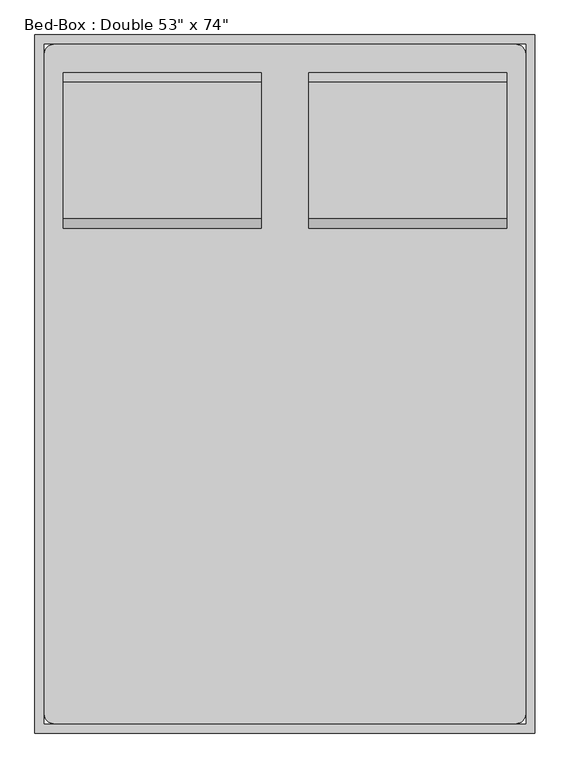
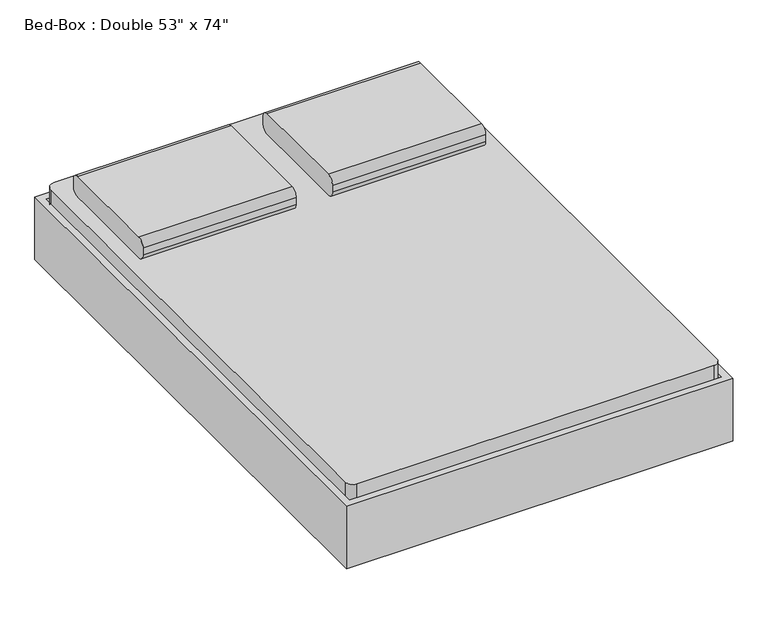
"""IFC4 building model written with IfcOpenShell, lengths in millimetres: furniture geometry."""

from ifc_helpers import new_model, si_unit, point, frame, frame_2d, origin, place, context, project, spatial, polyline, circle_curve, trimmed, segment, composite_curve, outline, extrude, source, transform, mapped, element, save
from ifc_brep_helpers import plane_surface, cylinder_surface, revolved_surface, advanced_brep


def furniture_bd6c971a(model_context):
    return source(origin(), model_context, "Body", "SolidModel", [
        extrude(outline(composite_curve([segment(polyline([(578.3704918, 406.4), (210.0704918, 406.4)]), True, "CONTINUOUS"), segment(trimmed(circle_curve(frame_2d((210.0704918, 431.8)), 25.4), [point((210.0704918, 406.4))], [point((184.6704918, 431.8))], False, "CARTESIAN"), True, "CONTINUOUS"), segment(polyline([(184.6704918, 431.8), (184.6704918, 457.2)]), True, "CONTINUOUS"), segment(trimmed(circle_curve(frame_2d((210.0704918, 457.2)), 25.4), [point((184.6704918, 457.2))], [point((210.0704918, 482.6))], False, "CARTESIAN"), True, "CONTINUOUS"), segment(polyline([(210.0704918, 482.6), (578.3704918, 482.6)]), True, "CONTINUOUS"), segment(trimmed(circle_curve(frame_2d((578.3704918, 457.2)), 25.4), [point((578.3704918, 482.6))], [point((603.7704918, 457.2))], False, "CARTESIAN"), True, "CONTINUOUS"), segment(polyline([(603.7704918, 457.2), (603.7704918, 431.8)]), True, "CONTINUOUS"), segment(trimmed(circle_curve(frame_2d((578.3704918, 431.8)), 25.4), [point((603.7704918, 431.8))], [point((578.3704918, 406.4))], False, "CARTESIAN"), True, "CONTINUOUS")], self_intersect=False)), frame((402.652459, 0.0, 0.0), z_axis=(1.0, 0.0, 0.0), x_axis=(0.0, 1.0, 0.0)), (0.0, 0.0, 1.0), 533.4),
        extrude(outline(composite_curve([segment(polyline([(578.3704918, 406.4), (210.0704918, 406.4)]), True, "CONTINUOUS"), segment(trimmed(circle_curve(frame_2d((210.0704918, 431.8)), 25.4), [point((210.0704918, 406.4))], [point((184.6704918, 431.8))], False, "CARTESIAN"), True, "CONTINUOUS"), segment(polyline([(184.6704918, 431.8), (184.6704918, 457.2)]), True, "CONTINUOUS"), segment(trimmed(circle_curve(frame_2d((210.0704918, 457.2)), 25.4), [point((184.6704918, 457.2))], [point((210.0704918, 482.6))], False, "CARTESIAN"), True, "CONTINUOUS"), segment(polyline([(210.0704918, 482.6), (578.3704918, 482.6)]), True, "CONTINUOUS"), segment(trimmed(circle_curve(frame_2d((578.3704918, 457.2)), 25.4), [point((578.3704918, 482.6))], [point((603.7704918, 457.2))], False, "CARTESIAN"), True, "CONTINUOUS"), segment(polyline([(603.7704918, 457.2), (603.7704918, 431.8)]), True, "CONTINUOUS"), segment(trimmed(circle_curve(frame_2d((578.3704918, 431.8)), 25.4), [point((603.7704918, 431.8))], [point((578.3704918, 406.4))], False, "CARTESIAN"), True, "CONTINUOUS")], self_intersect=False)), frame((-257.747541, 0.0, 0.0), z_axis=(1.0, 0.0, 0.0), x_axis=(0.0, 1.0, 0.0)), (0.0, 0.0, 1.0), 533.4),
        advanced_brep(
        [(-308.2231784, 451.3704918, 177.8), (-308.2231784, 375.1704918, 177.8), (-308.2231784, 375.1704918, 196.85), (-308.2231784, 451.3704918, 196.85), (-257.4231784, 451.3704918, 177.8), (-257.4231784, 375.1704918, 177.8), (-245.2869899, 375.1704918, 196.85), (-245.2869899, 451.3704918, 196.85), (-181.3523099, 451.3704918, 14.6654962), (-181.3523099, 375.1704918, 14.6654962), (-164.0871466, 375.1704918, 22.716374), (-164.0871466, 451.3704918, 22.716374), (-158.3320921, 375.1704918, 0.0), (-158.3320921, 451.3704918, 0.0), (-158.3320921, 375.1704918, 19.05), (-158.3320921, 451.3704918, 19.05), (-79.7195862, 451.3704918, 0.0), (-79.7195862, 375.1704918, 0.0), (-79.7195862, 375.1704918, 19.05), (-79.7195862, 451.3704918, 19.05), (-67.0195862, 375.1704918, 3.4029547), (-67.0195862, 451.3704918, 3.4029547), (-76.5445862, 375.1704918, 19.9007387), (-76.5445862, 451.3704918, 19.9007387), (-6.922541, 451.3704918, 38.1), (-6.922541, 375.1704918, 38.1), (-12.0269731, 375.1704918, 57.15), (-12.0269731, 451.3704918, 57.15), (685.5518216, 451.3704918, 38.1), (685.5518216, 375.1704918, 38.1), (690.6562537, 375.1704918, 57.15), (690.6562537, 451.3704918, 57.15), (745.6488669, 451.3704918, 3.4029547), (745.6488669, 375.1704918, 3.4029547), (755.1738669, 375.1704918, 19.9007387), (755.1738669, 451.3704918, 19.9007387), (758.3488669, 375.1704918, 0.0), (758.3488669, 451.3704918, 0.0), (758.3488669, 375.1704918, 19.05), (758.3488669, 451.3704918, 19.05), (836.9613728, 451.3704918, 0.0), (836.9613728, 375.1704918, 0.0), (836.9613728, 375.1704918, 19.05), (836.9613728, 451.3704918, 19.05), (859.9815906, 375.1704918, 14.6654962), (859.9815906, 451.3704918, 14.6654962), (842.7164272, 375.1704918, 22.716374), (842.7164272, 451.3704918, 22.716374), (936.052459, 451.3704918, 177.8), (936.052459, 375.1704918, 177.8), (923.9162705, 375.1704918, 196.85), (923.9162705, 451.3704918, 196.85), (986.852459, 451.3704918, 177.8), (986.852459, 451.3704918, 196.85), (986.852459, 375.1704918, 196.85), (986.852459, 375.1704918, 177.8)],
        [
            (0, 1),
            (1, 2),
            (2, 3),
            (3, 0),
            (0, 4),
            (4, 5),
            (5, 1),
            (5, 6),
            (6, 2),
            (6, 7),
            (7, 3),
            (7, 4),
            (4, 8),
            (8, 9),
            (9, 5),
            (9, 10),
            (10, 6),
            (10, 11),
            (11, 7),
            (11, 8),
            (12, 9, circle_curve(frame((-158.3320921, 375.1704918, 25.4), z_axis=(0.0, 1.0, 0.0), x_axis=(-0.9063077870366486, 0.0, -0.42261826174070233)), 25.4)),
            (8, 13, circle_curve(frame((-158.3320921, 451.3704918, 25.4), z_axis=(0.0, -1.0, 0.0), x_axis=(-0.9063077870366486, 0.0, -0.42261826174070233)), 25.4)),
            (13, 12),
            (14, 10, circle_curve(frame((-158.3320921, 375.1704918, 25.4), z_axis=(0.0, 1.0, 0.0), x_axis=(-0.9063077870366486, 0.0, -0.42261826174070233)), 6.35)),
            (12, 14),
            (15, 11, circle_curve(frame((-158.3320921, 451.3704918, 25.4), z_axis=(0.0, 1.0, 0.0), x_axis=(-0.9063077870366486, 0.0, -0.42261826174070233)), 6.35)),
            (14, 15),
            (15, 13),
            (13, 16),
            (16, 17),
            (17, 12),
            (17, 18),
            (18, 14),
            (18, 19),
            (19, 15),
            (19, 16),
            (20, 17, circle_curve(frame((-79.7195862, 375.1704918, 25.4), z_axis=(0.0, 1.0, 0.0), x_axis=(0.0, 0.0, -1.0)), 25.4)),
            (16, 21, circle_curve(frame((-79.7195862, 451.3704918, 25.4), z_axis=(0.0, -1.0, 0.0), x_axis=(0.0, 0.0, -1.0)), 25.4)),
            (21, 20),
            (22, 18, circle_curve(frame((-79.7195862, 375.1704918, 25.4), z_axis=(0.0, 1.0, 0.0), x_axis=(0.0, 0.0, -1.0)), 6.35)),
            (20, 22),
            (23, 19, circle_curve(frame((-79.7195862, 451.3704918, 25.4), z_axis=(0.0, 1.0, 0.0), x_axis=(0.0, 0.0, -1.0)), 6.35)),
            (22, 23),
            (23, 21),
            (21, 24),
            (24, 25),
            (25, 20),
            (25, 26),
            (26, 22),
            (26, 27),
            (27, 23),
            (27, 24),
            (24, 28),
            (28, 29),
            (29, 25),
            (29, 30),
            (30, 26),
            (30, 31),
            (31, 27),
            (31, 28),
            (28, 32),
            (32, 33),
            (33, 29),
            (33, 34),
            (34, 30),
            (34, 35),
            (35, 31),
            (35, 32),
            (36, 33, circle_curve(frame((758.3488669, 375.1704918, 25.4), z_axis=(0.0, 1.0, 0.0), x_axis=(-0.5000000000000463, 0.0, -0.8660254037844118)), 25.4)),
            (32, 37, circle_curve(frame((758.3488669, 451.3704918, 25.4), z_axis=(0.0, -1.0, 0.0), x_axis=(-0.5000000000000463, 0.0, -0.8660254037844118)), 25.4)),
            (37, 36),
            (38, 34, circle_curve(frame((758.3488669, 375.1704918, 25.4), z_axis=(0.0, 1.0, 0.0), x_axis=(-0.5000000000000463, 0.0, -0.8660254037844118)), 6.35)),
            (36, 38),
            (39, 35, circle_curve(frame((758.3488669, 451.3704918, 25.4), z_axis=(0.0, 1.0, 0.0), x_axis=(-0.5000000000000463, 0.0, -0.8660254037844118)), 6.35)),
            (38, 39),
            (39, 37),
            (37, 40),
            (40, 41),
            (41, 36),
            (41, 42),
            (42, 38),
            (42, 43),
            (43, 39),
            (43, 40),
            (44, 41, circle_curve(frame((836.9613728, 375.1704918, 25.4), z_axis=(0.0, 1.0, 0.0), x_axis=(0.0, 0.0, -1.0)), 25.4)),
            (40, 45, circle_curve(frame((836.9613728, 451.3704918, 25.4), z_axis=(0.0, -1.0, 0.0), x_axis=(0.0, 0.0, -1.0)), 25.4)),
            (45, 44),
            (46, 42, circle_curve(frame((836.9613728, 375.1704918, 25.4), z_axis=(0.0, 1.0, 0.0), x_axis=(0.0, 0.0, -1.0)), 6.35)),
            (44, 46),
            (47, 43, circle_curve(frame((836.9613728, 451.3704918, 25.4), z_axis=(0.0, 1.0, 0.0), x_axis=(0.0, 0.0, -1.0)), 6.35)),
            (46, 47),
            (47, 45),
            (45, 48),
            (48, 49),
            (49, 44),
            (49, 50),
            (50, 46),
            (50, 51),
            (51, 47),
            (51, 48),
            (52, 53),
            (53, 54),
            (54, 55),
            (55, 52),
            (48, 52),
            (55, 49),
            (54, 50),
            (53, 51),
        ],
        [
            plane_surface(frame((-308.2231784, 705.3704918, -152.9490627), z_axis=(-1.0, 0.0, 0.0), x_axis=(0.0, 1.0, 0.0))),
            plane_surface(frame((-308.2231784, 451.3704918, 177.8), z_axis=(0.0, 0.0, -1.0), x_axis=(1.0, 0.0, 0.0))),
            plane_surface(frame((-308.2231784, 375.1704918, 177.8), z_axis=(0.0, -1.0, 0.0), x_axis=(1.0, 0.0, 0.0))),
            plane_surface(frame((-308.2231784, 375.1704918, 196.85), z_axis=(0.0, 0.0, 1.0), x_axis=(1.0, 0.0, 0.0))),
            plane_surface(frame((-308.2231784, 451.3704918, 196.85), z_axis=(0.0, 1.0, 0.0), x_axis=(1.0, 0.0, 0.0))),
            plane_surface(frame((-257.4231784, 451.3704918, 177.8), z_axis=(-0.9063077870366488, 0.0, -0.42261826174070194), x_axis=(0.42261826174070194, 0.0, -0.9063077870366488))),
            plane_surface(frame((-257.4231784, 375.1704918, 177.8), z_axis=(0.0, -1.0, 0.0), x_axis=(0.42261826174070194, 0.0, -0.9063077870366488))),
            plane_surface(frame((-245.2869899, 375.1704918, 196.85), z_axis=(0.9063077870366487, 0.0, 0.4226182617407021), x_axis=(0.4226182617407021, 0.0, -0.9063077870366487))),
            plane_surface(frame((-245.2869899, 451.3704918, 196.85), z_axis=(0.0, 1.0, 0.0), x_axis=(0.4226182617407021, 0.0, -0.9063077870366487))),
            cylinder_surface(frame((-158.3320921, 705.3704918, 25.4), z_axis=(0.0, -1.0, 0.0), x_axis=(-0.9063077870366486, 0.0, -0.42261826174070233)), 25.4),
            plane_surface(frame((-158.3320921, 375.1704918, 25.4), z_axis=(0.0, -1.0, 0.0), x_axis=(-0.9063077870366486, 0.0, -0.42261826174070233))),
            revolved_surface(polyline([(-164.08714654768272, 375.1704918, 22.71637403794654), (-164.08714654768272, 451.3704918, 22.71637403794654)]), (-158.3320921, 705.3704918, 25.4), (0.0, -1.0, 0.0)),
            plane_surface(frame((-158.3320921, 451.3704918, 25.4), z_axis=(0.0, 1.0, 0.0), x_axis=(-0.9063077870366486, 0.0, -0.42261826174070233))),
            plane_surface(frame((-158.3320921, 451.3704918, 0.0), z_axis=(0.0, 0.0, -1.0), x_axis=(1.0, 0.0, 0.0))),
            plane_surface(frame((-158.3320921, 375.1704918, 0.0), z_axis=(0.0, -1.0, 0.0), x_axis=(1.0, 0.0, 0.0))),
            plane_surface(frame((-158.3320921, 375.1704918, 19.05), z_axis=(0.0, 0.0, 1.0), x_axis=(1.0, 0.0, 0.0))),
            plane_surface(frame((-158.3320921, 451.3704918, 19.05), z_axis=(0.0, 1.0, 0.0), x_axis=(1.0, 0.0, 0.0))),
            cylinder_surface(frame((-79.7195862, 705.3704918, 25.4), z_axis=(0.0, -1.0, 0.0), x_axis=(0.0, 0.0, -1.0)), 25.4),
            plane_surface(frame((-79.7195862, 375.1704918, 25.4), z_axis=(0.0, -1.0, 0.0), x_axis=(0.0, 0.0, -1.0))),
            revolved_surface(polyline([(-79.7195862, 375.1704918, 19.049999999999997), (-79.7195862, 451.3704918, 19.049999999999997)]), (-79.7195862, 705.3704918, 25.4), (0.0, -1.0, 0.0)),
            plane_surface(frame((-79.7195862, 451.3704918, 25.4), z_axis=(0.0, 1.0, 0.0), x_axis=(0.0, 0.0, -1.0))),
            plane_surface(frame((-67.0195862, 451.3704918, 3.4029547), z_axis=(0.4999999999998774, 0.0, -0.8660254037845095), x_axis=(0.8660254037845095, 0.0, 0.4999999999998774))),
            plane_surface(frame((-67.0195862, 375.1704918, 3.4029547), z_axis=(0.0, -1.0, 0.0), x_axis=(0.866025403784509, 0.0, 0.49999999999987815))),
            plane_surface(frame((-76.5445862, 375.1704918, 19.9007387), z_axis=(-0.49999999999987754, 0.0, 0.8660254037845093), x_axis=(0.8660254037845093, 0.0, 0.49999999999987754))),
            plane_surface(frame((-76.5445862, 451.3704918, 19.9007387), z_axis=(0.0, 1.0000000000000002, 0.0), x_axis=(0.8660254037845091, 0.0, 0.49999999999987815))),
            plane_surface(frame((-6.922541, 451.3704918, 38.1), z_axis=(0.0, 0.0, -1.0), x_axis=(1.0, 0.0, 0.0))),
            plane_surface(frame((-6.922541, 375.1704918, 38.1), z_axis=(0.0, -1.0, 0.0), x_axis=(1.0, 0.0, 0.0))),
            plane_surface(frame((-12.0269731, 375.1704918, 57.15), z_axis=(0.0, 0.0, 1.0), x_axis=(1.0, 0.0, 0.0))),
            plane_surface(frame((-12.0269731, 451.3704918, 57.15), z_axis=(0.0, 1.0, 0.0), x_axis=(1.0, 0.0, 0.0))),
            plane_surface(frame((685.5518216, 451.3704918, 38.1), z_axis=(-0.500000000000047, 0.0, -0.8660254037844115), x_axis=(0.8660254037844115, 0.0, -0.500000000000047))),
            plane_surface(frame((685.5518216, 375.1704918, 38.1), z_axis=(0.0, -1.0, 0.0), x_axis=(0.8660254037844116, 0.0, -0.500000000000047))),
            plane_surface(frame((690.6562537, 375.1704918, 57.15), z_axis=(0.5000000000000456, 0.0, 0.8660254037844124), x_axis=(0.8660254037844124, 0.0, -0.5000000000000456))),
            plane_surface(frame((690.6562537, 451.3704918, 57.15), z_axis=(0.0, 1.0, 0.0), x_axis=(0.8660254037844124, 0.0, -0.5000000000000456))),
            cylinder_surface(frame((758.3488669, 705.3704918, 25.4), z_axis=(0.0, -1.0, 0.0), x_axis=(-0.5000000000000463, 0.0, -0.8660254037844118)), 25.4),
            plane_surface(frame((758.3488669, 375.1704918, 25.4), z_axis=(0.0, -1.0000000000000002, 0.0), x_axis=(-0.5000000000000464, 0.0, -0.866025403784412))),
            revolved_surface(polyline([(755.1738668999997, 375.1704918, 19.90073868596898), (755.1738668999997, 451.3704918, 19.90073868596898)]), (758.3488669, 705.3704918, 25.4), (0.0, -1.0, 0.0)),
            plane_surface(frame((758.3488669, 451.3704918, 25.4), z_axis=(0.0, 1.0000000000000002, 0.0), x_axis=(-0.5000000000000464, 0.0, -0.866025403784412))),
            plane_surface(frame((758.3488669, 451.3704918, 0.0), z_axis=(0.0, 0.0, -1.0), x_axis=(1.0, 0.0, 0.0))),
            plane_surface(frame((758.3488669, 375.1704918, 0.0), z_axis=(0.0, -1.0, 0.0), x_axis=(1.0, 0.0, 0.0))),
            plane_surface(frame((758.3488669, 375.1704918, 19.05), z_axis=(0.0, 0.0, 1.0), x_axis=(1.0, 0.0, 0.0))),
            plane_surface(frame((758.3488669, 451.3704918, 19.05), z_axis=(0.0, 1.0, 0.0), x_axis=(1.0, 0.0, 0.0))),
            cylinder_surface(frame((836.9613728, 705.3704918, 25.4), z_axis=(0.0, -1.0, 0.0), x_axis=(0.0, 0.0, -1.0)), 25.4),
            plane_surface(frame((836.9613728, 375.1704918, 25.4), z_axis=(0.0, -1.0, 0.0), x_axis=(0.0, 0.0, -1.0))),
            revolved_surface(polyline([(836.9613728, 375.1704918, 19.049999999999997), (836.9613728, 451.3704918, 19.049999999999997)]), (836.9613728, 705.3704918, 25.4), (0.0, -1.0, 0.0)),
            plane_surface(frame((836.9613728, 451.3704918, 25.4), z_axis=(0.0, 1.0, 0.0), x_axis=(0.0, 0.0, -1.0))),
            plane_surface(frame((859.9815906, 451.3704918, 14.6654962), z_axis=(0.9063077870366798, 0.0, -0.4226182617406355), x_axis=(0.4226182617406355, 0.0, 0.9063077870366798))),
            plane_surface(frame((859.9815906, 375.1704918, 14.6654962), z_axis=(0.0, -1.0, 0.0), x_axis=(0.4226182617406356, 0.0, 0.9063077870366797))),
            plane_surface(frame((842.7164272, 375.1704918, 22.716374), z_axis=(-0.9063077870366797, 0.0, 0.4226182617406358), x_axis=(0.4226182617406358, 0.0, 0.9063077870366797))),
            plane_surface(frame((842.7164272, 451.3704918, 22.716374), z_axis=(0.0, 1.0000000000000002, 0.0), x_axis=(0.42261826174063544, 0.0, 0.9063077870366799))),
            plane_surface(frame((986.852459, 705.3704918, -152.9490627), z_axis=(1.0, 0.0, 0.0), x_axis=(0.0, 1.0, 0.0))),
            plane_surface(frame((936.052459, 451.3704918, 177.8), z_axis=(0.0, 0.0, -1.0), x_axis=(1.0, 0.0, 0.0))),
            plane_surface(frame((936.052459, 375.1704918, 177.8), z_axis=(0.0, -1.0, 0.0), x_axis=(1.0, 0.0, 0.0))),
            plane_surface(frame((923.9162705, 375.1704918, 196.85), z_axis=(0.0, 0.0, 1.0), x_axis=(1.0, 0.0, 0.0))),
            plane_surface(frame((923.9162705, 451.3704918, 196.85), z_axis=(0.0, 1.0, 0.0), x_axis=(1.0, 0.0, 0.0))),
        ],
        [
            (0, [[1, 2, 3, 4]]),
            (1, [[-1, 5, 6, 7]]),
            (2, [[-2, -7, 8, 9]]),
            (3, [[-3, -9, 10, 11]]),
            (4, [[-4, -11, 12, -5]]),
            (5, [[-6, 13, 14, 15]]),
            (6, [[-8, -15, 16, 17]]),
            (7, [[-10, -17, 18, 19]]),
            (8, [[-12, -19, 20, -13]]),
            (9, [[21, -14, 22, 23]]),
            (10, [[24, -16, -21, 25]]),
            (11, [[26, -18, -24, 27]]),
            (12, [[-22, -20, -26, 28]]),
            (13, [[-23, 29, 30, 31]]),
            (14, [[-25, -31, 32, 33]]),
            (15, [[-27, -33, 34, 35]]),
            (16, [[-28, -35, 36, -29]]),
            (17, [[37, -30, 38, 39]]),
            (18, [[40, -32, -37, 41]]),
            (19, [[42, -34, -40, 43]]),
            (20, [[-38, -36, -42, 44]]),
            (21, [[-39, 45, 46, 47]]),
            (22, [[-41, -47, 48, 49]]),
            (23, [[-43, -49, 50, 51]]),
            (24, [[-44, -51, 52, -45]]),
            (25, [[-46, 53, 54, 55]]),
            (26, [[-48, -55, 56, 57]]),
            (27, [[-50, -57, 58, 59]]),
            (28, [[-52, -59, 60, -53]]),
            (29, [[-54, 61, 62, 63]]),
            (30, [[-56, -63, 64, 65]]),
            (31, [[-58, -65, 66, 67]]),
            (32, [[-60, -67, 68, -61]]),
            (33, [[69, -62, 70, 71]]),
            (34, [[72, -64, -69, 73]]),
            (35, [[74, -66, -72, 75]]),
            (36, [[-70, -68, -74, 76]]),
            (37, [[-71, 77, 78, 79]]),
            (38, [[-73, -79, 80, 81]]),
            (39, [[-75, -81, 82, 83]]),
            (40, [[-76, -83, 84, -77]]),
            (41, [[85, -78, 86, 87]]),
            (42, [[88, -80, -85, 89]]),
            (43, [[90, -82, -88, 91]]),
            (44, [[-86, -84, -90, 92]]),
            (45, [[-87, 93, 94, 95]]),
            (46, [[-89, -95, 96, 97]]),
            (47, [[-91, -97, 98, 99]]),
            (48, [[-92, -99, 100, -93]]),
            (49, [[101, 102, 103, 104]]),
            (50, [[-94, 105, -104, 106]]),
            (51, [[-96, -106, -103, 107]]),
            (52, [[-98, -107, -102, 108]]),
            (53, [[-100, -108, -101, -105]]),
        ],
    ),
        extrude(outline(composite_curve([segment(polyline([(-283.147541, 679.9704918), (961.452459, 679.9704918)]), True, "CONTINUOUS"), segment(trimmed(circle_curve(frame_2d((961.452459, 654.5704918)), 25.4), [point((961.452459, 679.9704918))], [point((986.852459, 654.5704918))], False, "CARTESIAN"), True, "CONTINUOUS"), segment(polyline([(986.852459, 654.5704918), (986.852459, -1123.4295082)]), True, "CONTINUOUS"), segment(trimmed(circle_curve(frame_2d((961.452459, -1123.4295082)), 25.4), [point((986.852459, -1123.4295082))], [point((961.452459, -1148.8295082))], False, "CARTESIAN"), True, "CONTINUOUS"), segment(polyline([(961.452459, -1148.8295082), (-283.147541, -1148.8295082)]), True, "CONTINUOUS"), segment(trimmed(circle_curve(frame_2d((-283.147541, -1123.4295082)), 25.4), [point((-283.147541, -1148.8295082))], [point((-308.547541, -1123.4295082))], False, "CARTESIAN"), True, "CONTINUOUS"), segment(polyline([(-308.547541, -1123.4295082), (-308.547541, 654.5704918)]), True, "CONTINUOUS"), segment(trimmed(circle_curve(frame_2d((-283.147541, 654.5704918)), 25.4), [point((-308.547541, 654.5704918))], [point((-283.147541, 679.9704918))], False, "CARTESIAN"), True, "CONTINUOUS")], self_intersect=False)), frame((0.0, 0.0, 203.2), z_axis=(0.0, 0.0, 1.0), x_axis=(1.0, 0.0, 0.0)), (0.0, 0.0, 1.0), 203.2),
        advanced_brep(
        [(-308.547541, -869.4295082, 196.85), (-308.547541, -869.4295082, 177.8), (-308.547541, -945.6295082, 177.8), (-308.547541, -945.6295082, 196.85), (-245.6113525, -869.4295082, 196.85), (-257.747541, -869.4295082, 177.8), (-257.747541, -945.6295082, 177.8), (-245.6113525, -945.6295082, 196.85), (-164.4115092, -869.4295082, 22.716374), (-181.6766725, -869.4295082, 14.6654962), (-181.6766725, -945.6295082, 14.6654962), (-164.4115092, -945.6295082, 22.716374), (-158.6564547, -869.4295082, 0.0), (-158.6564547, -869.4295082, 19.05), (-158.6564547, -945.6295082, 0.0), (-158.6564547, -945.6295082, 19.05), (-80.0439489, -869.4295082, 19.05), (-80.0439489, -869.4295082, 0.0), (-80.0439489, -945.6295082, 0.0), (-80.0439489, -945.6295082, 19.05), (-67.3439489, -869.4295082, 3.4029547), (-76.8689489, -869.4295082, 19.9007387), (-67.3439489, -945.6295082, 3.4029547), (-76.8689489, -945.6295082, 19.9007387), (-12.3513357, -869.4295082, 57.15), (-7.2469036, -869.4295082, 38.1), (-7.2469036, -945.6295082, 38.1), (-12.3513357, -945.6295082, 57.15), (690.6562537, -869.4295082, 57.15), (685.5518216, -869.4295082, 38.1), (685.5518216, -945.6295082, 38.1), (690.6562537, -945.6295082, 57.15), (755.1738669, -869.4295082, 19.9007387), (745.6488669, -869.4295082, 3.4029547), (745.6488669, -945.6295082, 3.4029547), (755.1738669, -945.6295082, 19.9007387), (758.3488669, -869.4295082, 0.0), (758.3488669, -869.4295082, 19.05), (758.3488669, -945.6295082, 0.0), (758.3488669, -945.6295082, 19.05), (836.9613728, -869.4295082, 19.05), (836.9613728, -869.4295082, 0.0), (836.9613728, -945.6295082, 0.0), (836.9613728, -945.6295082, 19.05), (859.9815906, -869.4295082, 14.6654962), (842.7164272, -869.4295082, 22.716374), (859.9815906, -945.6295082, 14.6654962), (842.7164272, -945.6295082, 22.716374), (923.9162705, -869.4295082, 196.85), (936.052459, -869.4295082, 177.8), (936.052459, -945.6295082, 177.8), (923.9162705, -945.6295082, 196.85), (986.852459, -869.4295082, 196.85), (986.852459, -945.6295082, 196.85), (986.852459, -945.6295082, 177.8), (986.852459, -869.4295082, 177.8)],
        [
            (0, 1),
            (1, 2),
            (2, 3),
            (3, 0),
            (0, 4),
            (4, 5),
            (5, 1),
            (5, 6),
            (6, 2),
            (6, 7),
            (7, 3),
            (7, 4),
            (4, 8),
            (8, 9),
            (9, 5),
            (9, 10),
            (10, 6),
            (10, 11),
            (11, 7),
            (11, 8),
            (12, 9, circle_curve(frame((-158.6564547, -869.4295082, 25.4), z_axis=(0.0, 1.0, 0.0), x_axis=(-0.906307787036663, 0.0, -0.4226182617406713)), 25.4)),
            (8, 13, circle_curve(frame((-158.6564547, -869.4295082, 25.4), z_axis=(0.0, -1.0, 0.0), x_axis=(-0.906307787036663, 0.0, -0.4226182617406713)), 6.35)),
            (13, 12),
            (14, 10, circle_curve(frame((-158.6564547, -945.6295082, 25.4), z_axis=(0.0, 1.0, 0.0), x_axis=(-0.906307787036663, 0.0, -0.4226182617406713)), 25.4)),
            (12, 14),
            (15, 11, circle_curve(frame((-158.6564547, -945.6295082, 25.4), z_axis=(0.0, 1.0, 0.0), x_axis=(-0.906307787036663, 0.0, -0.4226182617406713)), 6.35)),
            (14, 15),
            (15, 13),
            (13, 16),
            (16, 17),
            (17, 12),
            (17, 18),
            (18, 14),
            (18, 19),
            (19, 15),
            (19, 16),
            (20, 17, circle_curve(frame((-80.0439489, -869.4295082, 25.4), z_axis=(0.0, 1.0, 0.0), x_axis=(0.0, 0.0, -1.0)), 25.4)),
            (16, 21, circle_curve(frame((-80.0439489, -869.4295082, 25.4), z_axis=(0.0, -1.0, 0.0), x_axis=(0.0, 0.0, -1.0)), 6.35)),
            (21, 20),
            (22, 18, circle_curve(frame((-80.0439489, -945.6295082, 25.4), z_axis=(0.0, 1.0, 0.0), x_axis=(0.0, 0.0, -1.0)), 25.4)),
            (20, 22),
            (23, 19, circle_curve(frame((-80.0439489, -945.6295082, 25.4), z_axis=(0.0, 1.0, 0.0), x_axis=(0.0, 0.0, -1.0)), 6.35)),
            (22, 23),
            (23, 21),
            (21, 24),
            (24, 25),
            (25, 20),
            (25, 26),
            (26, 22),
            (26, 27),
            (27, 23),
            (27, 24),
            (24, 28),
            (28, 29),
            (29, 25),
            (29, 30),
            (30, 26),
            (30, 31),
            (31, 27),
            (31, 28),
            (28, 32),
            (32, 33),
            (33, 29),
            (33, 34),
            (34, 30),
            (34, 35),
            (35, 31),
            (35, 32),
            (36, 33, circle_curve(frame((758.3488669, -869.4295082, 25.4), z_axis=(0.0, 1.0, 0.0), x_axis=(-0.5000000000000479, 0.0, -0.866025403784411)), 25.4)),
            (32, 37, circle_curve(frame((758.3488669, -869.4295082, 25.4), z_axis=(0.0, -1.0, 0.0), x_axis=(-0.5000000000000479, 0.0, -0.866025403784411)), 6.35)),
            (37, 36),
            (38, 34, circle_curve(frame((758.3488669, -945.6295082, 25.4), z_axis=(0.0, 1.0, 0.0), x_axis=(-0.5000000000000479, 0.0, -0.866025403784411)), 25.4)),
            (36, 38),
            (39, 35, circle_curve(frame((758.3488669, -945.6295082, 25.4), z_axis=(0.0, 1.0, 0.0), x_axis=(-0.5000000000000479, 0.0, -0.866025403784411)), 6.35)),
            (38, 39),
            (39, 37),
            (37, 40),
            (40, 41),
            (41, 36),
            (41, 42),
            (42, 38),
            (42, 43),
            (43, 39),
            (43, 40),
            (44, 41, circle_curve(frame((836.9613728, -869.4295082, 25.4), z_axis=(0.0, 1.0, 0.0), x_axis=(0.0, 0.0, -1.0)), 25.4)),
            (40, 45, circle_curve(frame((836.9613728, -869.4295082, 25.4), z_axis=(0.0, -1.0, 0.0), x_axis=(0.0, 0.0, -1.0)), 6.35)),
            (45, 44),
            (46, 42, circle_curve(frame((836.9613728, -945.6295082, 25.4), z_axis=(0.0, 1.0, 0.0), x_axis=(0.0, 0.0, -1.0)), 25.4)),
            (44, 46),
            (47, 43, circle_curve(frame((836.9613728, -945.6295082, 25.4), z_axis=(0.0, 1.0, 0.0), x_axis=(0.0, 0.0, -1.0)), 6.35)),
            (46, 47),
            (47, 45),
            (45, 48),
            (48, 49),
            (49, 44),
            (49, 50),
            (50, 46),
            (50, 51),
            (51, 47),
            (51, 48),
            (52, 53),
            (53, 54),
            (54, 55),
            (55, 52),
            (48, 52),
            (55, 49),
            (54, 50),
            (53, 51),
        ],
        [
            plane_surface(frame((-308.547541, -1174.2295082, -127.5947323), z_axis=(-1.0, 0.0, 0.0), x_axis=(0.0, 1.0, 0.0))),
            plane_surface(frame((-308.547541, -869.4295082, 196.85), z_axis=(0.0, 1.0, 0.0), x_axis=(1.0, 0.0, 0.0))),
            plane_surface(frame((-308.547541, -869.4295082, 177.8), z_axis=(0.0, 0.0, -1.0), x_axis=(1.0, 0.0, 0.0))),
            plane_surface(frame((-308.547541, -945.6295082, 177.8), z_axis=(0.0, -1.0, 0.0), x_axis=(1.0, 0.0, 0.0))),
            plane_surface(frame((-308.547541, -945.6295082, 196.85), z_axis=(0.0, 0.0, 1.0), x_axis=(1.0, 0.0, 0.0))),
            plane_surface(frame((-245.6113525, -869.4295082, 196.85), z_axis=(0.0, 1.0, 0.0), x_axis=(0.422618261740671, 0.0, -0.9063077870366633))),
            plane_surface(frame((-257.747541, -869.4295082, 177.8), z_axis=(-0.9063077870366631, 0.0, -0.42261826174067113), x_axis=(0.42261826174067113, 0.0, -0.9063077870366631))),
            plane_surface(frame((-257.747541, -945.6295082, 177.8), z_axis=(0.0, -1.0, 0.0), x_axis=(0.42261826174067135, 0.0, -0.906307787036663))),
            plane_surface(frame((-245.6113525, -945.6295082, 196.85), z_axis=(0.9063077870366631, 0.0, 0.4226182617406713), x_axis=(0.4226182617406713, 0.0, -0.9063077870366631))),
            plane_surface(frame((-158.6564547, -869.4295082, 25.4), z_axis=(0.0, 1.0, 0.0), x_axis=(-0.906307787036663, 0.0, -0.4226182617406713))),
            cylinder_surface(frame((-158.6564547, -1174.2295082, 25.4), z_axis=(0.0, -1.0, 0.0), x_axis=(-0.906307787036663, 0.0, -0.4226182617406713)), 25.4),
            plane_surface(frame((-158.6564547, -945.6295082, 25.4), z_axis=(0.0, -1.0, 0.0), x_axis=(-0.906307787036663, 0.0, -0.4226182617406713))),
            revolved_surface(polyline([(-164.41150914768284, -945.6295082, 22.716374037946736), (-164.41150914768284, -869.4295082, 22.716374037946736)]), (-158.6564547, -1174.2295082, 25.4), (0.0, -1.0, 0.0)),
            plane_surface(frame((-158.6564547, -869.4295082, 19.05), z_axis=(0.0, 1.0, 0.0), x_axis=(1.0, 0.0, 0.0))),
            plane_surface(frame((-158.6564547, -869.4295082, 0.0), z_axis=(0.0, 0.0, -1.0), x_axis=(1.0, 0.0, 0.0))),
            plane_surface(frame((-158.6564547, -945.6295082, 0.0), z_axis=(0.0, -1.0, 0.0), x_axis=(1.0, 0.0, 0.0))),
            plane_surface(frame((-158.6564547, -945.6295082, 19.05), z_axis=(0.0, 0.0, 1.0), x_axis=(1.0, 0.0, 0.0))),
            plane_surface(frame((-80.0439489, -869.4295082, 25.4), z_axis=(0.0, 1.0, 0.0), x_axis=(0.0, 0.0, -1.0))),
            cylinder_surface(frame((-80.0439489, -1174.2295082, 25.4), z_axis=(0.0, -1.0, 0.0), x_axis=(0.0, 0.0, -1.0)), 25.4),
            plane_surface(frame((-80.0439489, -945.6295082, 25.4), z_axis=(0.0, -1.0, 0.0), x_axis=(0.0, 0.0, -1.0))),
            revolved_surface(polyline([(-80.0439489, -945.6295082, 19.049999999999997), (-80.0439489, -869.4295082, 19.049999999999997)]), (-80.0439489, -1174.2295082, 25.4), (0.0, -1.0, 0.0)),
            plane_surface(frame((-76.8689489, -869.4295082, 19.9007387), z_axis=(0.0, 1.0, 0.0), x_axis=(0.8660254037844785, 0.0, 0.499999999999931))),
            plane_surface(frame((-67.3439489, -869.4295082, 3.4029547), z_axis=(0.499999999999931, 0.0, -0.8660254037844785), x_axis=(0.8660254037844785, 0.0, 0.499999999999931))),
            plane_surface(frame((-67.3439489, -945.6295082, 3.4029547), z_axis=(0.0, -1.0, 0.0), x_axis=(0.8660254037844786, 0.0, 0.49999999999993094))),
            plane_surface(frame((-76.8689489, -945.6295082, 19.9007387), z_axis=(-0.4999999999999312, 0.0, 0.8660254037844785), x_axis=(0.8660254037844785, 0.0, 0.4999999999999312))),
            plane_surface(frame((-12.3513357, -869.4295082, 57.15), z_axis=(0.0, 1.0, 0.0), x_axis=(1.0, 0.0, 0.0))),
            plane_surface(frame((-7.2469036, -869.4295082, 38.1), z_axis=(0.0, 0.0, -1.0), x_axis=(1.0, 0.0, 0.0))),
            plane_surface(frame((-7.2469036, -945.6295082, 38.1), z_axis=(0.0, -1.0, 0.0), x_axis=(1.0, 0.0, 0.0))),
            plane_surface(frame((-12.3513357, -945.6295082, 57.15), z_axis=(0.0, 0.0, 1.0), x_axis=(1.0, 0.0, 0.0))),
            plane_surface(frame((690.6562537, -869.4295082, 57.15), z_axis=(0.0, 1.0, 0.0), x_axis=(0.8660254037844091, 0.0, -0.5000000000000514))),
            plane_surface(frame((685.5518216, -869.4295082, 38.1), z_axis=(-0.5000000000000502, 0.0, -0.8660254037844097), x_axis=(0.8660254037844097, 0.0, -0.5000000000000502))),
            plane_surface(frame((685.5518216, -945.6295082, 38.1), z_axis=(0.0, -1.0, 0.0), x_axis=(0.86602540378441, 0.0, -0.5000000000000498))),
            plane_surface(frame((690.6562537, -945.6295082, 57.15), z_axis=(0.5000000000000505, 0.0, 0.8660254037844095), x_axis=(0.8660254037844095, 0.0, -0.5000000000000505))),
            plane_surface(frame((758.3488669, -869.4295082, 25.4), z_axis=(0.0, 1.0000000000000002, 0.0), x_axis=(-0.500000000000048, 0.0, -0.8660254037844111))),
            cylinder_surface(frame((758.3488669, -1174.2295082, 25.4), z_axis=(0.0, -1.0, 0.0), x_axis=(-0.5000000000000479, 0.0, -0.866025403784411)), 25.4),
            plane_surface(frame((758.3488669, -945.6295082, 25.4), z_axis=(0.0, -1.0000000000000002, 0.0), x_axis=(-0.500000000000048, 0.0, -0.8660254037844111))),
            revolved_surface(polyline([(755.1738668999997, -945.6295082, 19.90073868596899), (755.1738668999997, -869.4295082, 19.90073868596899)]), (758.3488669, -1174.2295082, 25.4), (0.0, -1.0, 0.0)),
            plane_surface(frame((758.3488669, -869.4295082, 19.05), z_axis=(0.0, 1.0, 0.0), x_axis=(1.0, 0.0, 0.0))),
            plane_surface(frame((758.3488669, -869.4295082, 0.0), z_axis=(0.0, 0.0, -1.0), x_axis=(1.0, 0.0, 0.0))),
            plane_surface(frame((758.3488669, -945.6295082, 0.0), z_axis=(0.0, -1.0, 0.0), x_axis=(1.0, 0.0, 0.0))),
            plane_surface(frame((758.3488669, -945.6295082, 19.05), z_axis=(0.0, 0.0, 1.0), x_axis=(1.0, 0.0, 0.0))),
            plane_surface(frame((836.9613728, -869.4295082, 25.4), z_axis=(0.0, 1.0, 0.0), x_axis=(0.0, 0.0, -1.0))),
            cylinder_surface(frame((836.9613728, -1174.2295082, 25.4), z_axis=(0.0, -1.0, 0.0), x_axis=(0.0, 0.0, -1.0)), 25.4),
            plane_surface(frame((836.9613728, -945.6295082, 25.4), z_axis=(0.0, -1.0, 0.0), x_axis=(0.0, 0.0, -1.0))),
            revolved_surface(polyline([(836.9613728, -945.6295082, 19.049999999999997), (836.9613728, -869.4295082, 19.049999999999997)]), (836.9613728, -1174.2295082, 25.4), (0.0, -1.0, 0.0)),
            plane_surface(frame((842.7164272, -869.4295082, 22.716374), z_axis=(0.0, 1.0, 0.0), x_axis=(0.4226182617405411, 0.0, 0.9063077870367238))),
            plane_surface(frame((859.9815906, -869.4295082, 14.6654962), z_axis=(0.9063077870367237, 0.0, -0.42261826174054157), x_axis=(0.42261826174054157, 0.0, 0.9063077870367237))),
            plane_surface(frame((859.9815906, -945.6295082, 14.6654962), z_axis=(0.0, -1.0, 0.0), x_axis=(0.4226182617405412, 0.0, 0.9063077870367238))),
            plane_surface(frame((842.7164272, -945.6295082, 22.716374), z_axis=(-0.906307787036724, 0.0, 0.422618261740541), x_axis=(0.422618261740541, 0.0, 0.906307787036724))),
            plane_surface(frame((986.852459, -1174.2295082, -127.5947323), z_axis=(1.0, 0.0, 0.0), x_axis=(0.0, 1.0, 0.0))),
            plane_surface(frame((923.9162705, -869.4295082, 196.85), z_axis=(0.0, 1.0, 0.0), x_axis=(1.0, 0.0, 0.0))),
            plane_surface(frame((936.052459, -869.4295082, 177.8), z_axis=(0.0, 0.0, -1.0), x_axis=(1.0, 0.0, 0.0))),
            plane_surface(frame((936.052459, -945.6295082, 177.8), z_axis=(0.0, -1.0, 0.0), x_axis=(1.0, 0.0, 0.0))),
            plane_surface(frame((923.9162705, -945.6295082, 196.85), z_axis=(0.0, 0.0, 1.0), x_axis=(1.0, 0.0, 0.0))),
        ],
        [
            (0, [[1, 2, 3, 4]]),
            (1, [[-1, 5, 6, 7]]),
            (2, [[-2, -7, 8, 9]]),
            (3, [[-3, -9, 10, 11]]),
            (4, [[-4, -11, 12, -5]]),
            (5, [[-6, 13, 14, 15]]),
            (6, [[-8, -15, 16, 17]]),
            (7, [[-10, -17, 18, 19]]),
            (8, [[-12, -19, 20, -13]]),
            (9, [[21, -14, 22, 23]]),
            (10, [[24, -16, -21, 25]]),
            (11, [[26, -18, -24, 27]]),
            (12, [[-22, -20, -26, 28]]),
            (13, [[-23, 29, 30, 31]]),
            (14, [[-25, -31, 32, 33]]),
            (15, [[-27, -33, 34, 35]]),
            (16, [[-28, -35, 36, -29]]),
            (17, [[37, -30, 38, 39]]),
            (18, [[40, -32, -37, 41]]),
            (19, [[42, -34, -40, 43]]),
            (20, [[-38, -36, -42, 44]]),
            (21, [[-39, 45, 46, 47]]),
            (22, [[-41, -47, 48, 49]]),
            (23, [[-43, -49, 50, 51]]),
            (24, [[-44, -51, 52, -45]]),
            (25, [[-46, 53, 54, 55]]),
            (26, [[-48, -55, 56, 57]]),
            (27, [[-50, -57, 58, 59]]),
            (28, [[-52, -59, 60, -53]]),
            (29, [[-54, 61, 62, 63]]),
            (30, [[-56, -63, 64, 65]]),
            (31, [[-58, -65, 66, 67]]),
            (32, [[-60, -67, 68, -61]]),
            (33, [[69, -62, 70, 71]]),
            (34, [[72, -64, -69, 73]]),
            (35, [[74, -66, -72, 75]]),
            (36, [[-70, -68, -74, 76]]),
            (37, [[-71, 77, 78, 79]]),
            (38, [[-73, -79, 80, 81]]),
            (39, [[-75, -81, 82, 83]]),
            (40, [[-76, -83, 84, -77]]),
            (41, [[85, -78, 86, 87]]),
            (42, [[88, -80, -85, 89]]),
            (43, [[90, -82, -88, 91]]),
            (44, [[-86, -84, -90, 92]]),
            (45, [[-87, 93, 94, 95]]),
            (46, [[-89, -95, 96, 97]]),
            (47, [[-91, -97, 98, 99]]),
            (48, [[-92, -99, 100, -93]]),
            (49, [[101, 102, 103, 104]]),
            (50, [[-94, 105, -104, 106]]),
            (51, [[-96, -106, -103, 107]]),
            (52, [[-98, -107, -102, 108]]),
            (53, [[-100, -108, -101, -105]]),
        ],
    ),
        extrude(outline(polyline([(1012.252459, 705.3704918), (1012.252459, -1174.2295082), (-333.947541, -1174.2295082), (-333.947541, 705.3704918), (1012.252459, 705.3704918)]), holes=[polyline([(986.852459, 679.9704918), (-308.547541, 679.9704918), (-308.547541, -1148.8295082), (986.852459, -1148.8295082), (986.852459, 679.9704918)])]), frame((0.0, 0.0, 127.0), z_axis=(0.0, 0.0, 1.0), x_axis=(1.0, 0.0, 0.0)), (0.0, 0.0, 1.0), 228.6),
    ])


if __name__ == "__main__":
    model = new_model("IFC4")
    model_context = context("Model", 3, world=origin())
    ifc_project = project(units=[si_unit("LENGTHUNIT", "METRE", prefix="MILLI")], contexts=[model_context])
    site = spatial("IfcSite", under=ifc_project)
    building = spatial("IfcBuilding", under=site)
    placement = place(None, origin())
    furniture_shape = furniture_bd6c971a(model_context)
    element("IfcFurniture", 1, ObjectType="Bed-Box : Double 53\" x 74\"", at=placement, inside=building, context=model_context, shape_type="MappedRepresentation", body=[
        mapped(furniture_shape, transform((0.0, 0.0, 0.0), x_axis=(1.0, 0.0, 0.0), y_axis=(0.0, 1.0, 0.0), z_axis=(0.0, 0.0, 1.0))),
    ])
    save(model, "model.ifc")

# Revit data of these elements
# Type "Bed-Box : Double 53\" x 74\""
#   Assembly Code = "E2020200"
#   Length = 6' - 2"
#   Width = 4' - 5"
#   Frame Material = Birch
#   Mattress Material = Linen, White
# Element 1 (IfcFurniture, "Bed-Box : Double 53\" x 74\"")
#   Materials on its faces: "Birch", "Linen, White"
# Materials
#   "Birch": class "Wood", colour RGB 224 178 126, transparency 0, Description = "Betula Alleghaniensis", Cost = 0
#   "Linen, White": class "Textile", colour RGB 247 247 239, transparency 0, Description = "Linen, white", Cost = 0
